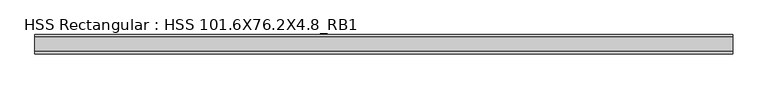
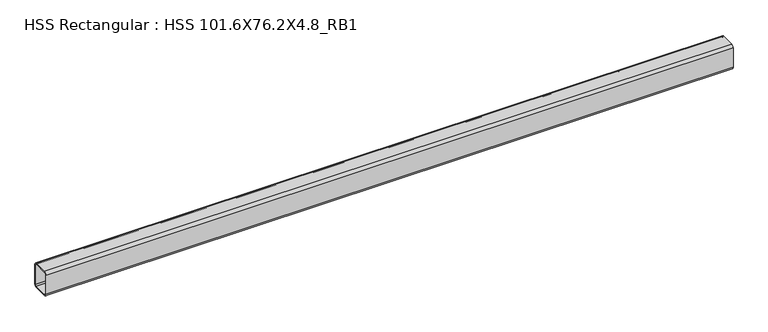
"""IFC4 building model written with IfcOpenShell, lengths in millimetres: beam geometry, HSS Rectangular : HSS 101.6X76.2X4.8_RB1."""

from ifc_helpers import new_model, si_unit, point, frame, frame_2d, origin, place, context, project, spatial, polyline, circle_curve, trimmed, segment, composite_curve, outline, extrude, source, transform, mapped, element, save


def hss_rectangular_hss_101_6x76_2x4_8_rb1_2cf97ae4(model_context):
    return source(origin(), model_context, "Body", "SweptSolid", [
        extrude(outline(composite_curve([segment(trimmed(circle_curve(frame_2d((-28.575, 41.275)), 9.525), [point((-38.1, 41.275))], [point((-28.575, 50.8))], False, "CARTESIAN"), True, "CONTINUOUS"), segment(polyline([(-28.575, 50.8), (28.575, 50.8)]), True, "CONTINUOUS"), segment(trimmed(circle_curve(frame_2d((28.575, 41.275)), 9.525), [point((28.575, 50.8))], [point((38.1, 41.275))], False, "CARTESIAN"), True, "CONTINUOUS"), segment(polyline([(38.1, 41.275), (38.1, -41.275)]), True, "CONTINUOUS"), segment(trimmed(circle_curve(frame_2d((28.575, -41.275)), 9.525), [point((38.1, -41.275))], [point((28.575, -50.8))], False, "CARTESIAN"), True, "CONTINUOUS"), segment(polyline([(28.575, -50.8), (-28.575, -50.8)]), True, "CONTINUOUS"), segment(trimmed(circle_curve(frame_2d((-28.575, -41.275)), 9.525), [point((-28.575, -50.8))], [point((-38.1, -41.275))], False, "CARTESIAN"), True, "CONTINUOUS"), segment(polyline([(-38.1, -41.275), (-38.1, 41.275)]), True, "CONTINUOUS")], self_intersect=False), holes=[composite_curve([segment(polyline([(28.575, 46.0375), (-28.575, 46.0375)]), True, "CONTINUOUS"), segment(trimmed(circle_curve(frame_2d((-28.575, 41.275)), 4.7625), [point((-28.575, 46.0375))], [point((-33.3375, 41.275))], True, "CARTESIAN"), True, "CONTINUOUS"), segment(polyline([(-33.3375, 41.275), (-33.3375, -41.275)]), True, "CONTINUOUS"), segment(trimmed(circle_curve(frame_2d((-28.575, -41.275)), 4.7625), [point((-33.3375, -41.275))], [point((-28.575, -46.0375))], True, "CARTESIAN"), True, "CONTINUOUS"), segment(polyline([(-28.575, -46.0375), (28.575, -46.0375)]), True, "CONTINUOUS"), segment(trimmed(circle_curve(frame_2d((28.575, -41.275)), 4.7625), [point((28.575, -46.0375))], [point((33.3375, -41.275))], True, "CARTESIAN"), True, "CONTINUOUS"), segment(polyline([(33.3375, -41.275), (33.3375, 41.275)]), True, "CONTINUOUS"), segment(trimmed(circle_curve(frame_2d((28.575, 41.275)), 4.7625), [point((33.3375, 41.275))], [point((28.575, 46.0375))], True, "CARTESIAN"), True, "CONTINUOUS")], self_intersect=False)]), frame((-1385.225, 0.0, 0.0), z_axis=(1.0, 0.0, 0.0), x_axis=(0.0, 1.0, 0.0)), (0.0, 0.0, 1.0), 2770.45),
    ])


if __name__ == "__main__":
    model = new_model("IFC4")
    model_context = context("Model", 3, world=origin())
    ifc_project = project(units=[si_unit("LENGTHUNIT", "METRE", prefix="MILLI")], contexts=[model_context])
    site = spatial("IfcSite", under=ifc_project)
    building = spatial("IfcBuilding", under=site)
    placement = place(None, origin())
    hss_rectangular_hss_101_6x76_2x4_8_rb1_shape = hss_rectangular_hss_101_6x76_2x4_8_rb1_2cf97ae4(model_context)
    element("IfcBeam", 1, ObjectType="HSS Rectangular : HSS 101.6X76.2X4.8_RB1", at=placement, inside=building, context=model_context, shape_type="MappedRepresentation", body=[
        mapped(hss_rectangular_hss_101_6x76_2x4_8_rb1_shape, transform((0.0, 0.0, 0.0), x_axis=(1.0, 0.0, 0.0), y_axis=(0.0, 1.0, 0.0), z_axis=(0.0, 0.0, 1.0))),
    ])
    save(model, "model.ifc")

# Revit data of these elements
# Type "HSS Rectangular : HSS 101.6X76.2X4.8_RB1"
#   Section Name Key = "HSS 4X3X3/16"
#   Assembly Code = "B10"
#   Width = 7.62 cm
#   Wall Nominal Thickness = 0.4763 cm
#   Wall Design Thickness = 0.442 cm
#   Torsional Moment of Inertia = 260.561 cm⁴
#   Torsional Modulus = 61.2876 cm³
#   Section Area = 14.4516 cm²
#   Plastic Modulus weak axis = 40.3122 cm³
#   Plastic Modulus strong axis = 49.1612 cm³
#   Perimeter = 0.881482 m²/m
#   Outer Fillet = 0.9525 cm
#   Nominal Weight = 12.1285 kgf/m
#   Moment of Inertia weak axis = 131.529 cm⁴
#   Moment of Inertia strong axis = 205.202 cm⁴
#   Inner Fillet = 0.4763 cm
#   Height = 10.16 cm
#   Elastic Modulus weak axis = 34.4128 cm³
#   Elastic Modulus strong axis = 40.476 cm³
#   Centroid Vertical = 5.08 cm
#   Centroid Horizontal = 3.81 cm
#   Length [instance default] = 1524 mm
#   Structural Material [instance default] = Steel ASTM A500, Grade B, Rectangular and Square
#   Principal Axes Angle = 0
# Element 1 (IfcBeam, "HSS Rectangular : HSS 101.6X76.2X4.8_RB1")
#   Structural Material = Steel ASTM A992
#   Materials on its faces: "Steel ASTM A992"
# Materials
#   "Steel ASTM A500, Grade B, Rectangular and Square": class "Metal", colour RGB 199 199 199, transparency 0, Description = "Carbon steel", Cost = 0
#   "Steel ASTM A992": class "Metal", colour RGB 199 199 199, transparency 0, Description = "Structural steel 50ksi", Cost = 0
